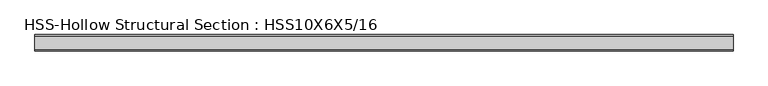
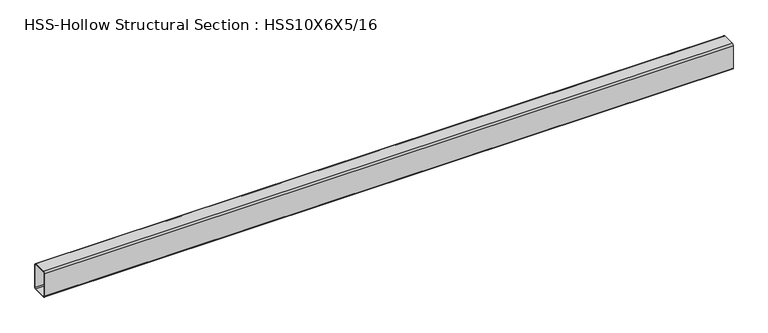
"""IFC4 building model written with IfcOpenShell, lengths in millimetres: beam geometry, HSS-Hollow Structural Section : HSS10X6X5/16."""

from ifc_helpers import new_model, si_unit, point, frame, frame_2d, origin, place, context, project, spatial, polyline, circle_curve, trimmed, segment, composite_curve, outline, extrude, source, transform, mapped, element, save


def hss_hollow_structural_section_hss10x6x5_16_ac06e8a8(model_context):
    return source(origin(), model_context, "Body", "SweptSolid", [
        extrude(outline(composite_curve([segment(polyline([(76.2, 112.2172), (76.2, -112.2172)]), True, "CONTINUOUS"), segment(trimmed(circle_curve(frame_2d((61.4172, -112.2172)), 14.7828), [point((76.2, -112.2172))], [point((61.4172, -127.0))], False, "CARTESIAN"), True, "CONTINUOUS"), segment(polyline([(61.4172, -127.0), (-61.4172, -127.0)]), True, "CONTINUOUS"), segment(trimmed(circle_curve(frame_2d((-61.4172, -112.2172)), 14.7828), [point((-61.4172, -127.0))], [point((-76.2, -112.2172))], False, "CARTESIAN"), True, "CONTINUOUS"), segment(polyline([(-76.2, -112.2172), (-76.2, 112.2172)]), True, "CONTINUOUS"), segment(trimmed(circle_curve(frame_2d((-61.4172, 112.2172)), 14.7828), [point((-76.2, 112.2172))], [point((-61.4172, 127.0))], False, "CARTESIAN"), True, "CONTINUOUS"), segment(polyline([(-61.4172, 127.0), (61.4172, 127.0)]), True, "CONTINUOUS"), segment(trimmed(circle_curve(frame_2d((61.4172, 112.2172)), 14.7828), [point((61.4172, 127.0))], [point((76.2, 112.2172))], False, "CARTESIAN"), True, "CONTINUOUS")], self_intersect=False), holes=[composite_curve([segment(trimmed(circle_curve(frame_2d((-61.4172, 112.2172)), 7.3914), [point((-61.4172, 119.6086))], [point((-68.8086, 112.2172))], True, "CARTESIAN"), True, "CONTINUOUS"), segment(polyline([(-68.8086, 112.2172), (-68.8086, -112.2172)]), True, "CONTINUOUS"), segment(trimmed(circle_curve(frame_2d((-61.4172, -112.2172)), 7.3914), [point((-68.8086, -112.2172))], [point((-61.4172, -119.6086))], True, "CARTESIAN"), True, "CONTINUOUS"), segment(polyline([(-61.4172, -119.6086), (61.4172, -119.6086)]), True, "CONTINUOUS"), segment(trimmed(circle_curve(frame_2d((61.4172, -112.2172)), 7.3914), [point((61.4172, -119.6086))], [point((68.8086, -112.2172))], True, "CARTESIAN"), True, "CONTINUOUS"), segment(polyline([(68.8086, -112.2172), (68.8086, 112.2172)]), True, "CONTINUOUS"), segment(trimmed(circle_curve(frame_2d((61.4172, 112.2172)), 7.3914), [point((68.8086, 112.2172))], [point((61.4172, 119.6086))], True, "CARTESIAN"), True, "CONTINUOUS"), segment(polyline([(61.4172, 119.6086), (-61.4172, 119.6086)]), True, "CONTINUOUS")], self_intersect=False)]), frame((-3299.5697009, 0.0, 0.0), z_axis=(1.0, 0.0, 0.0), x_axis=(0.0, 1.0, 0.0)), (0.0, 0.0, 1.0), 6510.6942979),
    ])


if __name__ == "__main__":
    model = new_model("IFC4")
    model_context = context("Model", 3, world=origin())
    ifc_project = project(units=[si_unit("LENGTHUNIT", "METRE", prefix="MILLI")], contexts=[model_context])
    site = spatial("IfcSite", under=ifc_project)
    building = spatial("IfcBuilding", under=site)
    placement = place(None, origin())
    hss_hollow_structural_section_hss10x6x5_16_shape = hss_hollow_structural_section_hss10x6x5_16_ac06e8a8(model_context)
    element("IfcBeam", 1, ObjectType="HSS-Hollow Structural Section : HSS10X6X5/16", at=placement, inside=building, context=model_context, shape_type="MappedRepresentation", body=[
        mapped(hss_hollow_structural_section_hss10x6x5_16_shape, transform((0.0, 0.0, 0.0), x_axis=(1.0, 0.0, 0.0), y_axis=(0.0, 1.0, 0.0), z_axis=(0.0, 0.0, 1.0))),
    ])
    save(model, "model.ifc")

# Revit data of these elements
# Type "HSS-Hollow Structural Section : HSS10X6X5/16"
#   Assembly Code = "B10"
#   Shape = "Rect."
#   W = 31.8
#   Ht = 0' - 10"
#   Length [instance default] = 5' - 0"
#   b = 0' - 6"
#   kr = 0' - 0.582"
#   t = 0' - 0.291"
#   A = 0.0608333 SF
#   Structural Material [instance default] = Steel ASTM A500, Grade B, Rectangular and Square
# Element 1 (IfcBeam, "HSS-Hollow Structural Section : HSS10X6X5/16")
#   Structural Material = Steel ASTM A992
#   Materials on its faces: "Steel ASTM A992"
# Materials
#   "Steel ASTM A500, Grade B, Rectangular and Square": class "Metal", colour RGB 199 199 199, transparency 0, Description = "Carbon steel", Cost = 0
#   "Steel ASTM A992": class "Metal", colour RGB 199 199 199, transparency 0, Description = "Structural steel 50ksi", Cost = 0
